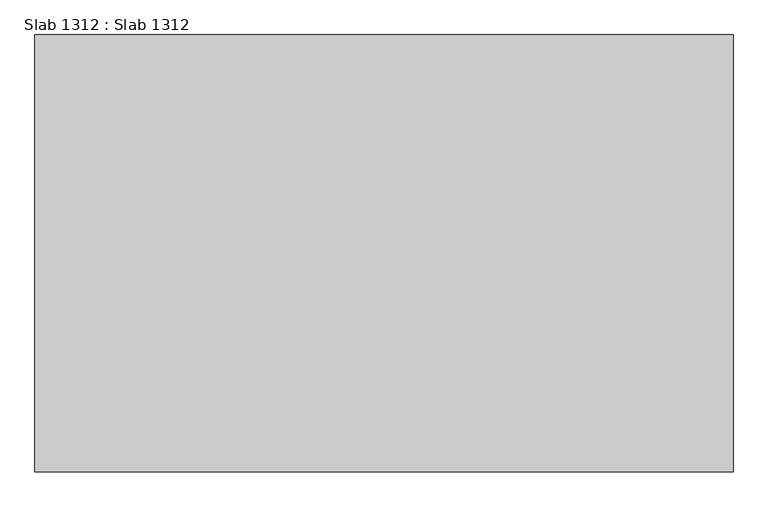
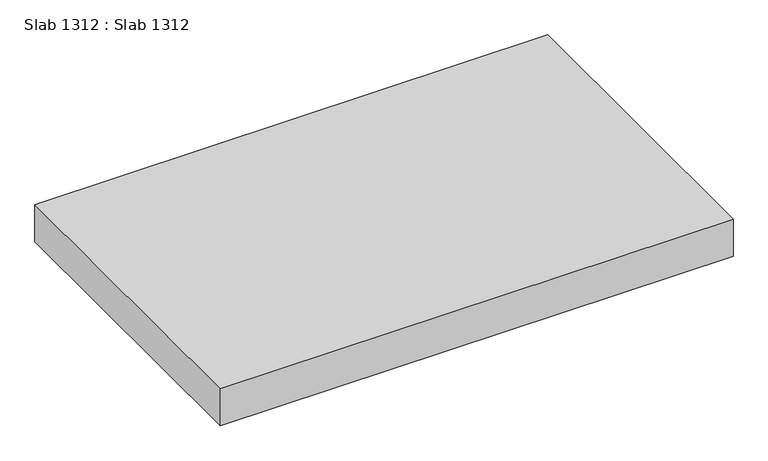
"""IFC4 building model written with IfcOpenShell, lengths in millimetres: proxy geometry, Slab 1312 : Slab 1312."""

from ifc_helpers import new_model, si_unit, frame, origin, place, context, project, spatial, polyline, outline, extrude, source, transform, mapped, element, save


def slab_1312_slab_1312_e76cee72(model_context):
    return source(origin(), model_context, "Body", "SweptSolid", [
        extrude(outline(polyline([(3694.2883192, 9744.3002787), (3694.2883192, 10997.0939628), (5694.2883192, 10997.0939628), (5694.2883192, 9744.3002787), (3694.2883192, 9744.3002787)])), frame((0.0, 0.0, 36175.6882407), z_axis=(0.0, 0.0, 1.0), x_axis=(1.0, 0.0, 0.0)), (0.0, 0.0, 1.0), 152.4077593),
    ])


if __name__ == "__main__":
    model = new_model("IFC4")
    model_context = context("Model", 3, world=origin())
    ifc_project = project(units=[si_unit("LENGTHUNIT", "METRE", prefix="MILLI")], contexts=[model_context])
    site = spatial("IfcSite", under=ifc_project)
    building = spatial("IfcBuilding", under=site)
    placement = place(None, origin())
    slab_1312_slab_1312_shape = slab_1312_slab_1312_e76cee72(model_context)
    element("IfcBuildingElementProxy", 1, Name="Slab 1312 : Slab 1312", ObjectType="Slab 1312 : Slab 1312", at=placement, inside=building, context=model_context, shape_type="MappedRepresentation", body=[
        mapped(slab_1312_slab_1312_shape, transform((0.0, 0.0, 0.0), x_axis=(1.0, 0.0, 0.0), y_axis=(0.0, 1.0, 0.0), z_axis=(0.0, 0.0, 1.0))),
    ])
    save(model, "model.ifc")

# Revit data of these elements
# Type "Slab 1312 : Slab 1312"
#   NameOverride = "Slab"
# Element 1 (IfcBuildingElementProxy, "Slab 1312 : Slab 1312")
#   Materials on its faces: "4\" CONCRETE SLAB - SEE CIVIL DWGS"
# Materials
#   "4\" CONCRETE SLAB - SEE CIVIL DWGS": class "Unassigned", colour RGB 128 128 128, transparency 0, Cost = 0
